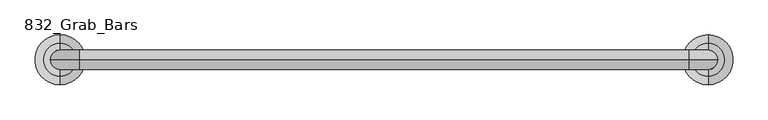
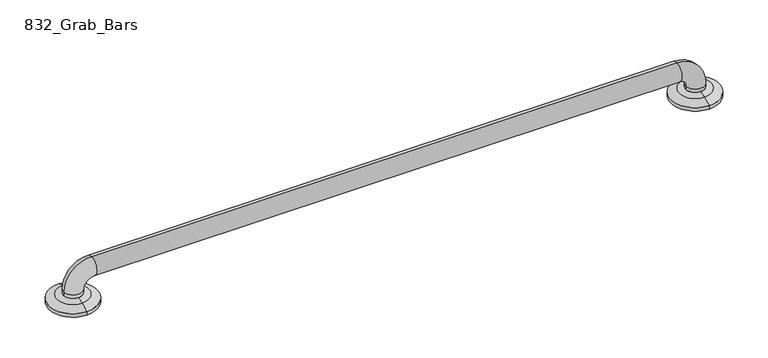
"""IFC4 building model written with IfcOpenShell, lengths in millimetres: proxy geometry, 832_Grab_Bars : 8320-001420."""

import ifcopenshell
import ifcopenshell.guid

model = None  # the IFC model being written
_history = None  # IfcOwnerHistory: only IFC2X3 demands one
_inside = {}  # id of a spatial element -> (the spatial element, [elements in it])
_under = {}  # id of a project, library or spatial element -> (it, [spatial elements below it])
_declared = {}  # id of a project -> (the project, [libraries it declares])
_typed = {}  # id of a type object -> (the type object, [elements of that type])
_made_of = {}  # id of a material, layer set ... -> (it, [elements and type objects made of it])


def new_model(schema):
    """Start an empty IFC model of exactly this schema.

    Asked for "IFC4X3", IfcOpenShell would pick the latest addendum, in which some entities
    have other attributes; the version numbers below select the first issue.
    IFC2X3 requires an IfcOwnerHistory on every rooted entity: one is made here for all.
    """
    global model, _history
    if schema == "IFC4X3":
        model = ifcopenshell.file(schema_version=(4, 3, 0, 0))
    else:
        model = ifcopenshell.file(schema=schema)
    _inside.clear()
    _under.clear()
    _declared.clear()
    _typed.clear()
    _made_of.clear()
    _history = None
    if model.schema == "IFC2X3":
        org = make("IfcOrganization", Name="unknown")
        user = make(
            "IfcPersonAndOrganization",
            ThePerson=make("IfcPerson", FamilyName="unknown"),
            TheOrganization=org,
        )
        app = make(
            "IfcApplication",
            ApplicationDeveloper=org,
            Version="unknown",
            ApplicationFullName="unknown",
            ApplicationIdentifier="unknown",
        )
        _history = make(
            "IfcOwnerHistory",
            OwningUser=user,
            OwningApplication=app,
            ChangeAction="ADDED",
            CreationDate=0,
        )
    return model


def make(cls, **values):
    """One entity of the class cls with the attributes given. An attribute that is None is left unset."""
    return model.create_entity(
        cls, **{name: value for name, value in values.items() if value is not None}
    )


def rooted(cls, **values):
    """An entity with a GlobalId (a new one), such as an element, a storey or a relation."""
    return make(cls, GlobalId=ifcopenshell.guid.new(), OwnerHistory=_history, **values)


def si_unit(unit_type, name, prefix=None):
    """IfcSIUnit, for example si_unit("LENGTHUNIT", "METRE", prefix="MILLI")."""
    return make("IfcSIUnit", UnitType=unit_type, Prefix=prefix, Name=name)


def assignment(units):
    """IfcUnitAssignment: the units of a project."""
    return None if units is None else make("IfcUnitAssignment", Units=units)


def point(xyz):
    """IfcCartesianPoint."""
    return None if xyz is None else make("IfcCartesianPoint", Coordinates=xyz)


def direction(xyz):
    """IfcDirection."""
    return None if xyz is None else make("IfcDirection", DirectionRatios=xyz)


def frame(location, z_axis=None, x_axis=None):
    """IfcAxis2Placement3D, a coordinate frame: its origin and axes. An axis left out is left unset."""
    return make(
        "IfcAxis2Placement3D",
        Location=point(location),
        Axis=direction(z_axis),
        RefDirection=direction(x_axis),
    )


def origin():
    """The frame at (0, 0, 0) with its axes left unset."""
    return frame((0.0, 0.0, 0.0))


def place(relative_to, where):
    """IfcLocalPlacement: puts the frame where relative to a parent placement (None: the world)."""
    return make(
        "IfcLocalPlacement", PlacementRelTo=relative_to, RelativePlacement=where
    )


def context(
    kind, dimensions, precision=None, world=None, true_north=None, identifier=None
):
    """IfcGeometricRepresentationContext, for example the 3D "Model" context."""
    return make(
        "IfcGeometricRepresentationContext",
        ContextIdentifier=identifier,
        ContextType=kind,
        CoordinateSpaceDimension=dimensions,
        Precision=precision,
        WorldCoordinateSystem=world,
        TrueNorth=true_north,
    )


def project(units=None, contexts=None):
    """IfcProject with its units and contexts."""
    return rooted(
        "IfcProject",
        Name="project",
        RepresentationContexts=contexts,
        UnitsInContext=assignment(units),
    )


def spatial(cls, under=None, at=None, **own):
    """A site, building, storey or space (cls), placed at a placement, below another one or the project."""
    s = rooted(cls, ObjectPlacement=at, **own)
    if under is not None:
        _under.setdefault(under.id(), (under, []))[1].append(s)
    return s


def polyline(points):
    """IfcPolyline through the points."""
    return make("IfcPolyline", Points=[point(p) for p in points])


def circle_curve(where, radius):
    """IfcCircle in the frame where."""
    return make("IfcCircle", Position=where, Radius=radius)


def ellipse_curve(where, semi_axis1, semi_axis2):
    """IfcEllipse in the frame where."""
    return make(
        "IfcEllipse", Position=where, SemiAxis1=semi_axis1, SemiAxis2=semi_axis2
    )


def trimmed(basis, trim1, trim2, sense, master):
    """IfcTrimmedCurve: the piece of a basis curve between two trims."""
    return make(
        "IfcTrimmedCurve",
        BasisCurve=basis,
        Trim1=trim1,
        Trim2=trim2,
        SenseAgreement=sense,
        MasterRepresentation=master,
    )


def shape(context_of_items, identifier, shape_type, items):
    """IfcShapeRepresentation: the items that make up one representation, for example the "Body"."""
    return make(
        "IfcShapeRepresentation",
        ContextOfItems=context_of_items,
        RepresentationIdentifier=identifier,
        RepresentationType=shape_type,
        Items=items,
    )


def source(mapping_origin, context_of_items, identifier, shape_type, items):
    """IfcRepresentationMap: a shape defined once, which mapped items show again and again."""
    return make(
        "IfcRepresentationMap",
        MappingOrigin=mapping_origin,
        MappedRepresentation=shape(context_of_items, identifier, shape_type, items),
    )


def transform(
    local_origin,
    x_axis=None,
    y_axis=None,
    z_axis=None,
    scale=None,
    scale2=None,
    scale3=None,
    uniform=True,
):
    """IfcCartesianTransformationOperator3D, or its non-uniform kind. x_axis, y_axis, z_axis: its Axis1, 2, 3."""
    if uniform:
        return make(
            "IfcCartesianTransformationOperator3D",
            Axis1=direction(x_axis),
            Axis2=direction(y_axis),
            LocalOrigin=point(local_origin),
            Scale=scale,
            Axis3=direction(z_axis),
        )
    return make(
        "IfcCartesianTransformationOperator3DnonUniform",
        Axis1=direction(x_axis),
        Axis2=direction(y_axis),
        LocalOrigin=point(local_origin),
        Scale=scale,
        Axis3=direction(z_axis),
        Scale2=scale2,
        Scale3=scale3,
    )


def mapped(mapping_source, mapping_target):
    """IfcMappedItem: shows the shape of a source again, moved by a transform."""
    return make(
        "IfcMappedItem", MappingSource=mapping_source, MappingTarget=mapping_target
    )


def made_of(thing, what):
    """Note that an element or type object is made of a material, layer set ...; save() writes the relation."""
    if what is not None:
        _made_of.setdefault(what.id(), (what, []))[1].append(thing)
    return thing


def element(
    cls,
    number,
    at=None,
    inside=None,
    cuts=None,
    type_object=None,
    material=None,
    context=None,
    identifier="Body",
    shape_type=None,
    held_by="IfcProductDefinitionShape",
    body=None,
    shapes=None,
    **own,
):
    """One element of the class cls, such as IfcWall. Its Tag is "e" and its number.

    at: its placement. inside: the storey or other place that contains it. cuts: it is an
    opening in that element (IfcRelVoidsElement). A single representation is given by context,
    identifier, shape_type and body (its items); several are given by shapes. held_by: the class
    of the entity that holds the representations. save() writes the other relations.
    """
    e = rooted(cls, Tag="e%d" % number, ObjectPlacement=at, **own)
    if body is not None:
        shapes = [shape(context, identifier, shape_type, body)]
    if shapes is not None:
        e.Representation = make(held_by, Representations=shapes)
    if inside is not None:
        _inside.setdefault(inside.id(), (inside, []))[1].append(e)
    if cuts is not None:
        rooted(
            "IfcRelVoidsElement", RelatingBuildingElement=cuts, RelatedOpeningElement=e
        )
    if type_object is not None:
        _typed.setdefault(type_object.id(), (type_object, []))[1].append(e)
    return made_of(e, material)


def aggregate(whole, parts):
    """IfcRelAggregates: a whole, such as a stair, and the parts it consists of."""
    return rooted("IfcRelAggregates", RelatingObject=whole, RelatedObjects=parts)


def save(model, path):
    """Write the relations noted so far, then the file.

    IfcRelAggregates (storeys below a building ...), IfcRelContainedInSpatialStructure (elements
    in a storey), IfcRelDefinesByType, IfcRelAssociatesMaterial and IfcRelDeclares: one each for
    every whole, place, type object, material and project.
    """
    for whole, parts in _under.values():
        aggregate(whole, parts)
    for where, things in _inside.values():
        rooted(
            "IfcRelContainedInSpatialStructure",
            RelatedElements=things,
            RelatingStructure=where,
        )
    for kind, things in _typed.values():
        rooted("IfcRelDefinesByType", RelatedObjects=things, RelatingType=kind)
    for what, things in _made_of.values():
        rooted("IfcRelAssociatesMaterial", RelatedObjects=things, RelatingMaterial=what)
    for by, libraries in _declared.values():
        rooted("IfcRelDeclares", RelatingContext=by, RelatedDefinitions=libraries)
    model.write(path)


def plane_surface(at):
    """IfcPlane: the flat surface through the origin of the frame at, square to its z axis."""
    return make("IfcPlane", Position=at)


def cylinder_surface(at, radius):
    """IfcCylindricalSurface: all points at the distance radius from the z axis of the frame at."""
    return make("IfcCylindricalSurface", Position=at, Radius=radius)


def revolved_surface(curve, axis_point, axis_direction):
    """IfcSurfaceOfRevolution: the curve turned about the line through axis_point along axis_direction."""
    return make(
        "IfcSurfaceOfRevolution",
        SweptCurve=make("IfcArbitraryOpenProfileDef", ProfileType="CURVE", Curve=curve),
        AxisPosition=make("IfcAxis1Placement", Location=point(axis_point), Axis=direction(axis_direction)),
    )


def advanced_brep(points, edges, surfaces, faces):
    """IfcAdvancedBrep: a solid bounded by faces that lie on surfaces and meet in shared edges.

    An edge is (start, end): straight between two places in points (the first is 0);
    or (start, end, curve); or (start, end, curve, False) where it runs against its curve.
    A face is (place in surfaces, loops), or (place, loops, False) where it looks against
    its surface's normal. A loop lists edges by number (the first is 1), with a minus sign
    where the edge is run from its end to its start. The first loop is the outer one.
    """
    corners = [point(p) for p in points]
    vertices = [make("IfcVertexPoint", VertexGeometry=c) for c in corners]
    made = []
    for start, end, *more in edges:
        made.append(
            make(
                "IfcEdgeCurve",
                EdgeStart=vertices[start],
                EdgeEnd=vertices[end],
                EdgeGeometry=more[0] if more else make("IfcPolyline", Points=[corners[start], corners[end]]),
                SameSense=more[1] if len(more) > 1 else True,
            )
        )
    hull = []
    for where, loops, *sense in faces:
        bounds = []
        for j, loop in enumerate(loops):
            ring = [make("IfcOrientedEdge", EdgeElement=made[abs(k) - 1], Orientation=k > 0) for k in loop]
            bounds.append(
                make(
                    "IfcFaceOuterBound" if j == 0 else "IfcFaceBound",
                    Bound=make("IfcEdgeLoop", EdgeList=ring),
                    Orientation=True,
                )
            )
        hull.append(make("IfcAdvancedFace", Bounds=bounds, FaceSurface=surfaces[where], SameSense=sense[0] if sense else True))
    return make("IfcAdvancedBrep", Outer=make("IfcClosedShell", CfsFaces=hull))


def proxy_832_grab_bars_99aa9c40(model_context):
    return source(origin(), model_context, "Body", "AdvancedBrep", [
        advanced_brep(
        [(-439.7375, -564.1630987, 13.1934507), (-439.7375, -508.9869013, 13.1934507), (-439.7375, -495.3, 6.35), (-439.7375, -577.85, 6.35), (-439.7375, -552.8038734, 15.875), (-439.7375, -520.3461266, 15.875), (-439.7375, -552.45, 15.875), (-455.6125, -536.575, 15.875), (-439.7375, -520.7, 15.875), (-423.8625, -536.575, 15.875), (-439.7375, -577.85, 0.0), (-439.7375, -495.3, 0.0), (-439.7375, -520.7, 0.0), (-439.7375, -536.575, 0.0), (-439.7375, -552.45, 0.0), (627.0625, -564.2276895, 13.1934507), (627.0625, -509.0514921, 13.1934507), (627.0625, -495.3645908, 6.35), (627.0625, -577.9145908, 6.35), (627.0625, -552.8684641, 15.875), (627.0625, -520.4107174, 15.875), (627.0625, -552.45, 15.875), (611.1875, -536.575, 15.875), (627.0625, -520.7, 15.875), (642.9375, -536.575, 15.875), (627.0625, -577.9145908, 0.0), (627.0625, -495.3645908, 0.0), (627.0625, -520.7, 0.0), (627.0625, -536.6395908, 0.0), (627.0625, -552.45, 0.0), (-455.6125, -536.575, 22.225), (-423.8625, -536.575, 22.225), (-407.9875, -536.575, 69.85), (-407.9875, -536.575, 38.1), (595.3125, -536.575, 69.85), (595.3125, -536.575, 38.1), (642.9375, -536.575, 22.225), (611.1875, -536.575, 22.225)],
        [
            (0, 1, circle_curve(frame((-439.7375, -536.575, 13.1934507), z_axis=(0.0, 0.0, -1.0), x_axis=(0.0, 1.0, 0.0)), 27.5880987)),
            (1, 2),
            (2, 3, circle_curve(frame((-439.7375, -536.575, 6.35), z_axis=(0.0, 0.0, 1.0), x_axis=(0.0, 1.0, 0.0)), 41.275)),
            (3, 0),
            (1, 0, circle_curve(frame((-439.7375, -536.575, 13.1934507), z_axis=(0.0, 0.0, -1.0), x_axis=(0.0, 1.0, 0.0)), 27.5880987)),
            (3, 2, circle_curve(frame((-439.7375, -536.575, 6.35), z_axis=(0.0, 0.0, 1.0), x_axis=(0.0, 1.0, 0.0)), 41.275)),
            (0, 4, circle_curve(frame((-439.7375, -552.8038734, -9.525), z_axis=(-1.0, 0.0, 0.0), x_axis=(0.0, 0.0, -1.0)), 25.4)),
            (4, 5, circle_curve(frame((-439.7375, -536.575, 15.875), z_axis=(0.0, 0.0, -1.0), x_axis=(0.0, 1.0, 0.0)), 16.2288734)),
            (5, 1, circle_curve(frame((-439.7375, -520.3461266, -9.525), z_axis=(-1.0, 0.0, 0.0), x_axis=(0.0, 0.0, -1.0)), 25.4)),
            (5, 4, circle_curve(frame((-439.7375, -536.575, 15.875), z_axis=(0.0, 0.0, -1.0), x_axis=(0.0, 1.0, 0.0)), 16.2288734)),
            (4, 6),
            (6, 7, circle_curve(frame((-439.7375, -536.575, 15.875), z_axis=(0.0, 0.0, -1.0), x_axis=(1.0, 0.0, 0.0)), 15.875)),
            (7, 8, circle_curve(frame((-439.7375, -536.575, 15.875), z_axis=(0.0, 0.0, -1.0), x_axis=(1.0, 0.0, 0.0)), 15.875)),
            (8, 5),
            (8, 9, circle_curve(frame((-439.7375, -536.575, 15.875), z_axis=(0.0, 0.0, -1.0), x_axis=(1.0, 0.0, 0.0)), 15.875)),
            (9, 6, circle_curve(frame((-439.7375, -536.575, 15.875), z_axis=(0.0, 0.0, -1.0), x_axis=(1.0, 0.0, 0.0)), 15.875)),
            (10, 11, circle_curve(frame((-439.7375, -536.575, 0.0), z_axis=(0.0, 0.0, -1.0), x_axis=(0.0, 1.0, 0.0)), 41.275)),
            (11, 12),
            (12, 13),
            (13, 14),
            (14, 10),
            (11, 10, circle_curve(frame((-439.7375, -536.575, 0.0), z_axis=(0.0, 0.0, -1.0), x_axis=(0.0, 1.0, 0.0)), 41.275)),
            (2, 11),
            (10, 3),
            (15, 16, circle_curve(frame((627.0625, -536.6395908, 13.1934507), z_axis=(0.0, 0.0, -1.0), x_axis=(0.0, 1.0, 0.0)), 27.5880987)),
            (16, 17),
            (17, 18, circle_curve(frame((627.0625, -536.6395908, 6.35), z_axis=(0.0, 0.0, 1.0), x_axis=(0.0, 1.0, 0.0)), 41.275)),
            (18, 15),
            (16, 15, circle_curve(frame((627.0625, -536.6395908, 13.1934507), z_axis=(0.0, 0.0, -1.0), x_axis=(0.0, 1.0, 0.0)), 27.5880987)),
            (18, 17, circle_curve(frame((627.0625, -536.6395908, 6.35), z_axis=(0.0, 0.0, 1.0), x_axis=(0.0, 1.0, 0.0)), 41.275)),
            (15, 19, circle_curve(frame((627.0625, -552.8684641, -9.525), z_axis=(-1.0, 0.0, 0.0), x_axis=(0.0, 0.0, -1.0)), 25.4)),
            (19, 20, circle_curve(frame((627.0625, -536.6395908, 15.875), z_axis=(0.0, 0.0, -1.0), x_axis=(0.0, 1.0, 0.0)), 16.2288734)),
            (20, 16, circle_curve(frame((627.0625, -520.4107174, -9.525), z_axis=(-1.0, 0.0, 0.0), x_axis=(0.0, 0.0, -1.0)), 25.4)),
            (20, 19, circle_curve(frame((627.0625, -536.6395908, 15.875), z_axis=(0.0, 0.0, -1.0), x_axis=(0.0, 1.0, 0.0)), 16.2288734)),
            (19, 21),
            (21, 22, circle_curve(frame((627.0625, -536.575, 15.875), z_axis=(0.0, 0.0, -1.0), x_axis=(-1.0, 0.0, 0.0)), 15.875)),
            (22, 23, circle_curve(frame((627.0625, -536.575, 15.875), z_axis=(0.0, 0.0, -1.0), x_axis=(-1.0, 0.0, 0.0)), 15.875)),
            (23, 20),
            (23, 24, circle_curve(frame((627.0625, -536.575, 15.875), z_axis=(0.0, 0.0, -1.0), x_axis=(-1.0, 0.0, 0.0)), 15.875)),
            (24, 21, circle_curve(frame((627.0625, -536.575, 15.875), z_axis=(0.0, 0.0, -1.0), x_axis=(-1.0, 0.0, 0.0)), 15.875)),
            (25, 26, circle_curve(frame((627.0625, -536.6395908, 0.0), z_axis=(0.0, 0.0, -1.0), x_axis=(0.0, 1.0, 0.0)), 41.275)),
            (26, 27),
            (27, 28),
            (28, 29),
            (29, 25),
            (26, 25, circle_curve(frame((627.0625, -536.6395908, 0.0), z_axis=(0.0, 0.0, -1.0), x_axis=(0.0, 1.0, 0.0)), 41.275)),
            (17, 26),
            (25, 18),
            (30, 31, circle_curve(frame((-439.7375, -536.575, 22.225), z_axis=(0.0, 0.0, -1.0), x_axis=(1.0, 0.0, 0.0)), 15.875)),
            (31, 9),
            (7, 30),
            (31, 30, circle_curve(frame((-439.7375, -536.575, 22.225), z_axis=(0.0, 0.0, -1.0), x_axis=(1.0, 0.0, 0.0)), 15.875)),
            (30, 32, circle_curve(frame((-407.9875, -536.575, 22.225), z_axis=(0.0, 1.0, 0.0), x_axis=(-1.0, 0.0, 0.0)), 47.625)),
            (32, 33, circle_curve(frame((-407.9875, -536.575, 53.975), z_axis=(-1.0, 0.0, 0.0), x_axis=(0.0, 0.0, -1.0)), 15.875)),
            (33, 31, circle_curve(frame((-407.9875, -536.575, 22.225), z_axis=(0.0, -1.0, 0.0), x_axis=(-1.0, 0.0, 0.0)), 15.875)),
            (33, 32, circle_curve(frame((-407.9875, -536.575, 53.975), z_axis=(-1.0, 0.0, 0.0), x_axis=(0.0, 0.0, -1.0)), 15.875)),
            (32, 34),
            (34, 35, circle_curve(frame((595.3125, -536.575, 53.975), z_axis=(-1.0, 0.0, 0.0), x_axis=(0.0, 0.0, -1.0)), 15.875)),
            (35, 33),
            (35, 34, circle_curve(frame((595.3125, -536.575, 53.975), z_axis=(-1.0, 0.0, 0.0), x_axis=(0.0, 0.0, -1.0)), 15.875)),
            (34, 36, circle_curve(frame((595.3125, -536.575, 22.225), z_axis=(0.0, 1.0, 0.0), x_axis=(0.0, 0.0, 1.0)), 47.625)),
            (36, 37, circle_curve(frame((627.0625, -536.575, 22.225), z_axis=(0.0, 0.0, 1.0), x_axis=(-1.0, 0.0, 0.0)), 15.875)),
            (37, 35, circle_curve(frame((595.3125, -536.575, 22.225), z_axis=(0.0, -1.0, 0.0), x_axis=(0.0, 0.0, 1.0)), 15.875)),
            (37, 36, circle_curve(frame((627.0625, -536.575, 22.225), z_axis=(0.0, 0.0, 1.0), x_axis=(-1.0, 0.0, 0.0)), 15.875)),
            (36, 24),
            (22, 37),
        ],
        [
            revolved_surface(polyline([(-439.7375, -495.3, 6.35), (-439.7375, -508.9869013, 13.1934507)]), (-439.7375, -536.575, 31.75), (0.0, 0.0, 1.0)),
            revolved_surface(trimmed(ellipse_curve(frame((-439.7375, -520.3461266, -9.525), z_axis=(1.0, 0.0, 0.0), x_axis=(0.0, 0.0, -1.0)), 25.4, 25.4), [point((-439.7375, -508.9869013, 13.1934507))], [point((-439.7375, -520.3461266, 15.875))], True, "CARTESIAN"), (-439.7375, -536.575, 31.75), (0.0, 0.0, 1.0)),
            plane_surface(frame((-439.7375, -536.575, 15.875), z_axis=(0.0, 0.0, 1.0), x_axis=(0.0, 1.0, 0.0))),
            plane_surface(frame((-439.7375, -536.575, 0.0), z_axis=(0.0, 0.0, -1.0), x_axis=(0.0, 1.0, 0.0))),
            cylinder_surface(frame((-439.7375, -536.575, 31.75), z_axis=(0.0, 0.0, 1.0), x_axis=(0.0, 1.0, 0.0)), 41.275),
            revolved_surface(polyline([(627.0625, -495.3645908, 6.35), (627.0625, -509.0514921, 13.1934507)]), (627.0625, -536.6395908, 31.75), (0.0, 0.0, 1.0)),
            revolved_surface(trimmed(ellipse_curve(frame((627.0625, -520.4107174, -9.525), z_axis=(1.0, 0.0, 0.0), x_axis=(0.0, 0.0, -1.0)), 25.4, 25.4), [point((627.0625, -509.0514921, 13.1934507))], [point((627.0625, -520.4107174, 15.875))], True, "CARTESIAN"), (627.0625, -536.6395908, 31.75), (0.0, 0.0, 1.0)),
            plane_surface(frame((627.0625, -536.6395908, 15.875), z_axis=(0.0, 0.0, 1.0), x_axis=(0.0, 1.0, 0.0))),
            plane_surface(frame((627.0625, -536.6395908, 0.0), z_axis=(0.0, 0.0, -1.0), x_axis=(0.0, 1.0, 0.0))),
            cylinder_surface(frame((627.0625, -536.6395908, 31.75), z_axis=(0.0, 0.0, 1.0), x_axis=(0.0, 1.0, 0.0)), 41.275),
            cylinder_surface(frame((-439.7375, -536.575, 0.0), z_axis=(0.0, 0.0, -1.0), x_axis=(1.0, 0.0, 0.0)), 15.875),
            revolved_surface(trimmed(ellipse_curve(frame((-439.7375, -536.575, 22.225), z_axis=(0.0, 0.0, -1.0), x_axis=(1.0, 0.0, 0.0)), 15.875, 15.875), [point((-455.6125, -536.575, 22.225))], [point((-423.8625, -536.575, 22.225))], True, "CARTESIAN"), (-407.9875, -536.575, 22.225), (0.0, 1.0, 0.0)),
            revolved_surface(trimmed(ellipse_curve(frame((-439.7375, -536.575, 22.225), z_axis=(0.0, 0.0, -1.0), x_axis=(1.0, 0.0, 0.0)), 15.875, 15.875), [point((-423.8625, -536.575, 22.225))], [point((-455.6125, -536.575, 22.225))], True, "CARTESIAN"), (-407.9875, -536.575, 22.225), (0.0, 1.0, 0.0)),
            cylinder_surface(frame((-407.9875, -536.575, 53.975), z_axis=(-1.0, 0.0, 0.0), x_axis=(0.0, 0.0, -1.0)), 15.875),
            revolved_surface(trimmed(ellipse_curve(frame((595.3125, -536.575, 53.975), z_axis=(-1.0, 0.0, 0.0), x_axis=(0.0, 0.0, -1.0)), 15.875, 15.875), [point((595.3125, -536.575, 69.85))], [point((595.3125, -536.575, 38.1))], True, "CARTESIAN"), (595.3125, -536.575, 22.225), (0.0, 1.0, 0.0)),
            revolved_surface(trimmed(ellipse_curve(frame((595.3125, -536.575, 53.975), z_axis=(-1.0, 0.0, 0.0), x_axis=(0.0, 0.0, -1.0)), 15.875, 15.875), [point((595.3125, -536.575, 38.1))], [point((595.3125, -536.575, 69.85))], True, "CARTESIAN"), (595.3125, -536.575, 22.225), (0.0, 1.0, 0.0)),
            cylinder_surface(frame((627.0625, -536.575, 22.225), z_axis=(0.0, 0.0, 1.0), x_axis=(-1.0, 0.0, 0.0)), 15.875),
        ],
        [
            (0, [[1, 2, 3, 4]]),
            (0, [[-2, 5, -4, 6]]),
            (1, [[-1, 7, 8, 9]]),
            (1, [[-5, -9, 10, -7]]),
            (2, [[-8, 11, 12, 13, 14]]),
            (2, [[-10, -14, 15, 16, -11]]),
            (3, [[17, 18, 19, 20, 21]]),
            (3, [[22, -21, -20, -19, -18]]),
            (4, [[-3, 23, -17, 24]]),
            (4, [[-6, -24, -22, -23]]),
            (5, [[25, 26, 27, 28]]),
            (5, [[-26, 29, -28, 30]]),
            (6, [[-25, 31, 32, 33]]),
            (6, [[-29, -33, 34, -31]]),
            (7, [[-32, 35, 36, 37, 38]]),
            (7, [[-34, -38, 39, 40, -35]]),
            (8, [[41, 42, 43, 44, 45]]),
            (8, [[46, -45, -44, -43, -42]]),
            (9, [[-27, 47, -41, 48]]),
            (9, [[-30, -48, -46, -47]]),
            (10, [[49, 50, -15, -13, 51]]),
            (10, [[52, -51, -12, -16, -50]]),
            (11, [[-49, 53, 54, 55]]),
            (12, [[-52, -55, 56, -53]]),
            (13, [[-54, 57, 58, 59]]),
            (13, [[-56, -59, 60, -57]]),
            (14, [[-58, 61, 62, 63]]),
            (15, [[-60, -63, 64, -61]]),
            (16, [[-62, 65, -39, -37, 66]]),
            (16, [[-64, -66, -36, -40, -65]]),
        ],
    ),
    ])


if __name__ == "__main__":
    model = new_model("IFC4")
    model_context = context("Model", 3, world=origin())
    ifc_project = project(units=[si_unit("LENGTHUNIT", "METRE", prefix="MILLI")], contexts=[model_context])
    site = spatial("IfcSite", under=ifc_project)
    building = spatial("IfcBuilding", under=site)
    placement = place(None, origin())
    proxy_832_grab_bars_shape = proxy_832_grab_bars_99aa9c40(model_context)
    element("IfcBuildingElementProxy", 1, Name="832_Grab_Bars : 8320-001420", ObjectType="832_Grab_Bars : 8320-001420", at=placement, inside=building, context=model_context, shape_type="MappedRepresentation", body=[
        mapped(proxy_832_grab_bars_shape, transform((0.0, 0.0, 0.0), x_axis=(1.0, 0.0, 0.0), y_axis=(0.0, 1.0, 0.0), z_axis=(0.0, 0.0, 1.0))),
    ])
    save(model, "model.ifc")

# Revit data of these elements
# Type "832_Grab_Bars : 8320-001420"
#   Warranty Information = "Complete unit, one (1) year"
#   Version = "1.0"
#   Technical Data = "http://www.bradleycorp.com/products/techdata/8820.pdf"
#   URL = "www.bradleycorp.com"
#   Type Comments = "All grab bar configurations are specified using centerline to centerline dimensions."
#   OmniClass Title = ""
#   Modeling Code = ""
#   Model = "8320-001420"
#   Material Note = "FLANGES - 13GA., ESCUTCHEONS - 22GA., TUBING - 18GA."
#   MasterFormat Section Title = ""
#   Manufacturer = "Bradley Corporation"
#   LEED Credit = ""
#   Instructions [instance default] = "This is a face mounted fixture."
#   Industry Standards = "ANSI Standard A117.1, ADA, ABA, ADAAG, UFAS"
#   Fire Rating = "None"
#   Description = "Grab Bars"
#   Copyright = "This Model Data is Property of Bradley Corporation"
#   Complies to NAFTA = "Yes"
#   Complies To Buy American Act = "Yes"
#   Assembly Code = "C1030200"
#   ADA Compliant = "Yes"
#   Radius = 15.875 mm
#   Percentage of Recycled Content = 64.98
#   Overall Length = 1149.35 mm
#   OmniClass Code = 0
#   MasterFormat Section Number = 0
#   Length = 1066.8 mm
#   Diameter = 31.75 mm
#   Default Elevation = 838.2 mm
#   Material and Finish = Bradley Corp Stainless Steel - Satin
# Element 1 (IfcBuildingElementProxy, "832_Grab_Bars : 8320-001420")
#   Materials on its faces: "Bradley Corp Stainless Steel - Satin"
# Materials
#   "Bradley Corp Stainless Steel - Satin": class "Metal", colour RGB 189 187 185, transparency 0, Manufacturer = "Bradley Corporation", URL = "www.bradleycorp.com", Description = "Stainless Steel - Satin Finish", Cost = 0
